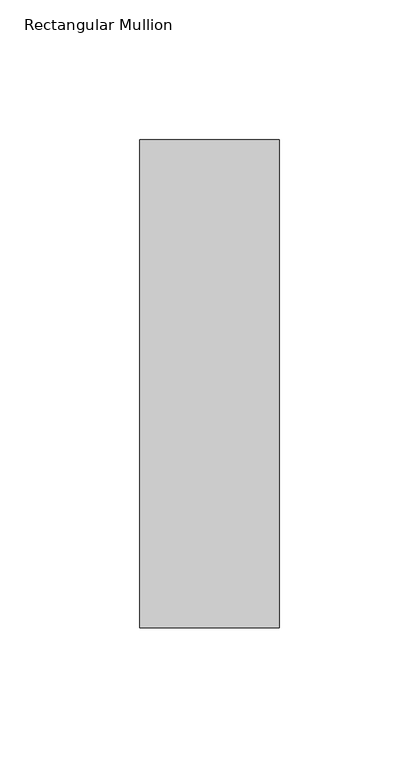
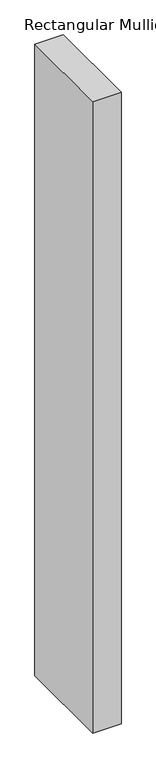
"""IFC4 building model written with IfcOpenShell, lengths in millimetres: member geometry, Rectangular Mullion : WWm-50x175-50mmOffset."""

from ifc_helpers import new_model, si_unit, frame, origin, place, context, project, spatial, polyline, outline, extrude, source, transform, mapped, element, save


def rectangular_mullion_b4814f12(model_context):
    return source(origin(), model_context, "Body", "SweptSolid", [
        extrude(outline(polyline([(0.0, 87.5), (0.0, -87.5), (-50.0, -87.5), (-50.0, 87.5), (0.0, 87.5)])), frame((0.0, 0.0, -1170.0), z_axis=(0.0, 0.0, 1.0), x_axis=(1.0, 0.0, 0.0)), (0.0, 0.0, 1.0), 1170.0),
    ])


if __name__ == "__main__":
    model = new_model("IFC4")
    model_context = context("Model", 3, world=origin())
    ifc_project = project(units=[si_unit("LENGTHUNIT", "METRE", prefix="MILLI")], contexts=[model_context])
    site = spatial("IfcSite", under=ifc_project)
    building = spatial("IfcBuilding", under=site)
    placement = place(None, origin())
    rectangular_mullion_shape = rectangular_mullion_b4814f12(model_context)
    element("IfcMember", 1, ObjectType="Rectangular Mullion : WWm-50x175-50mmOffset", at=placement, inside=building, context=model_context, shape_type="MappedRepresentation", body=[
        mapped(rectangular_mullion_shape, transform((0.0, 0.0, 0.0), x_axis=(1.0, 0.0, 0.0), y_axis=(0.0, 1.0, 0.0), z_axis=(0.0, 0.0, 1.0))),
    ])
    save(model, "model.ifc")

# Revit data of these elements
# Type "Rectangular Mullion : WWm-50x175-50mmOffset"
#   built-in parameter 1007304 = 0.574147 (stored number, unit not read)
#   built-in parameter 1007301 = 0.082021 (stored number, unit not read)
#   built-in parameter 1007300 = 0.082021 (stored number, unit not read)
# Element 1 (IfcMember, "Rectangular Mullion : WWm-50x175-50mmOffset")
#   Materials on its faces: "WW-EC-RGB-Mullion"
# Materials
#   "WW-EC-RGB-Mullion": class "Generic", colour RGB 255 255 255, transparency 0, Comments = "If region requests black mullions, switch asset color to RGB 25-25-25", Description = "Generic Color", Cost = 0
